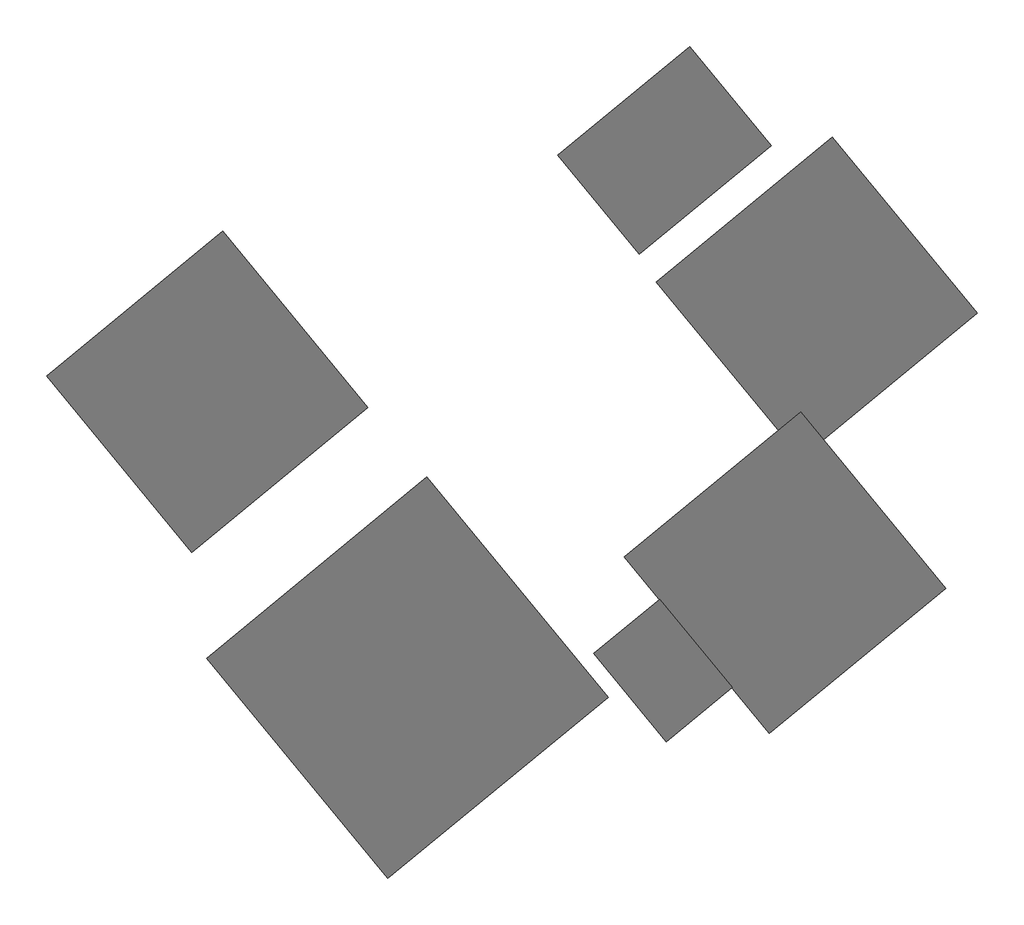
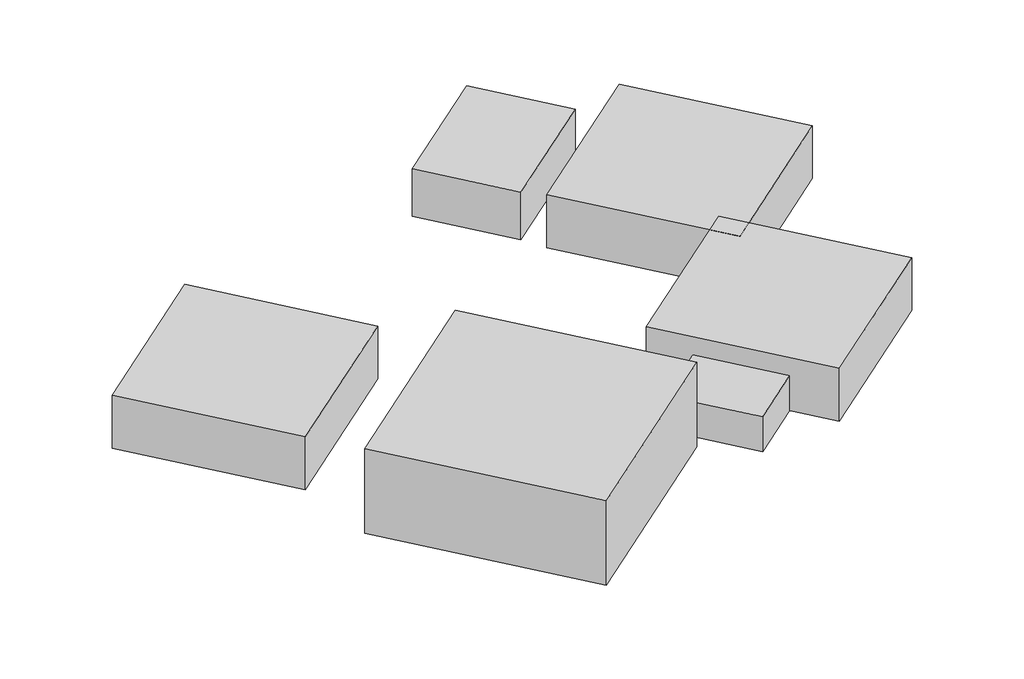
# One storey: 6 proxies.
"""IFC4 building model written with IfcOpenShell, lengths in millimetres."""

from ifc_helpers import new_model, si_unit, frame, origin, place, context, project, spatial, polyline, outline, extrude, element, save

model = new_model("IFC4")

# Units and contexts
model_context = context("Model", 3, world=origin())
ifc_project = project(units=[si_unit("LENGTHUNIT", "METRE", prefix="MILLI")], contexts=[model_context])

# Site, building, storey
site = spatial("IfcSite", under=ifc_project)
building = spatial("IfcBuilding", under=site)
storey = spatial("IfcBuildingStorey", under=building, Name="f3-展厅", Elevation=17500.0)

# Proxies
placement = place(None, origin())
element("IfcBuildingElementProxy", 1, Name="公共-封闭 : Gallery-Big", ObjectType="公共-封闭 : Gallery-Big", at=placement, inside=storey, context=model_context, shape_type="SweptSolid", body=[
    extrude(outline(polyline([(-29475.375386, -24866.8019738), (-42184.0405117, -9423.6860084), (-26740.9245463, 3284.9791173), (-14032.2594206, -12158.1368482), (-29475.375386, -24866.8019738)])), frame((0.0, 0.0, 17500.0), z_axis=(0.0, 0.0, 1.0), x_axis=(1.0, 0.0, 0.0)), (0.0, 0.0, 1.0), 8000.0),
])
element("IfcBuildingElementProxy", 2, Name="公共-封闭 : Gallery-Middle", ObjectType="公共-封闭 : Gallery-Middle", at=placement, inside=storey, context=model_context, shape_type="SweptSolid", body=[
    extrude(outline(polyline([(-492.5871713, 4613.457612), (-10659.5192719, 16967.9503844), (1694.9735005, 27134.8824849), (11861.9056011, 14780.3897125), (-492.5871713, 4613.457612)])), frame((0.0, 0.0, 17500.0), z_axis=(0.0, 0.0, 1.0), x_axis=(1.0, 0.0, 0.0)), (0.0, 0.0, 1.0), 5000.0),
])
element("IfcBuildingElementProxy", 3, Name="公共-封闭 : Gallery-Middle", ObjectType="公共-封闭 : Gallery-Middle", at=placement, inside=storey, context=model_context, shape_type="SweptSolid", body=[
    extrude(outline(polyline([(-2728.7186006, -14686.3227176), (-12895.6507012, -2331.8299452), (-541.1579288, 7835.1021553), (9625.7741718, -4519.3906171), (-2728.7186006, -14686.3227176)])), frame((0.0, 0.0, 17500.0), z_axis=(0.0, 0.0, 1.0), x_axis=(1.0, 0.0, 0.0)), (0.0, 0.0, 1.0), 5000.0),
])
element("IfcBuildingElementProxy", 4, Name="公共-封闭 : Gallery-Middle", ObjectType="公共-封闭 : Gallery-Middle", at=placement, inside=storey, context=model_context, shape_type="SweptSolid", body=[
    extrude(outline(polyline([(-43231.5828584, -1987.7462838), (-53398.514959, 10366.7464885), (-41044.0221866, 20533.6785891), (-30877.0900861, 8179.1858167), (-43231.5828584, -1987.7462838)])), frame((0.0, 0.0, 17500.0), z_axis=(0.0, 0.0, 1.0), x_axis=(1.0, 0.0, 0.0)), (0.0, 0.0, 1.0), 5000.0),
])
element("IfcBuildingElementProxy", 5, Name="公共-封闭 : Gallery-Small", ObjectType="公共-封闭 : Gallery-Small", at=placement, inside=storey, context=model_context, shape_type="SweptSolid", body=[
    extrude(outline(polyline([(-11856.9381005, 18909.0766924), (-17575.8374071, 25858.4788769), (-8309.9678278, 33483.6779523), (-2591.0685212, 26534.2757679), (-11856.9381005, 18909.0766924)])), frame((0.0, 0.0, 17500.0), z_axis=(0.0, 0.0, 1.0), x_axis=(1.0, 0.0, 0.0)), (0.0, 0.0, 1.0), 4500.0),
])
element("IfcBuildingElementProxy", 6, Name="临时私有-封闭 : Restrooms-Gallery-3f", ObjectType="临时私有-封闭 : Restrooms-Gallery-3f", at=placement, inside=storey, context=model_context, shape_type="SweptSolid", body=[
    extrude(outline(polyline([(-5312.0353372, -11458.3253572), (-9944.9701269, -15270.9248949), (-15028.4361772, -9093.6785087), (-10395.5013875, -5281.078971), (-5312.0353372, -11458.3253572)])), frame((0.0, 0.0, 17500.0), z_axis=(0.0, 0.0, 1.0), x_axis=(1.0, 0.0, 0.0)), (0.0, 0.0, 1.0), 3300.0),
])

save(model, "model.ifc")

# Revit data of these elements
# Type "公共-封闭 : Gallery-Big"
#   Default Elevation = 1219.2 mm
#   公共_封闭_房间_面积 = 400.00 m²
#   公共_封闭_房间_进深 = 20000 mm
#   公共_封闭_房间_开间 = 20000 mm
#   公共_封闭_房间_层高 = 8000 mm
# Type "公共-封闭 : Gallery-Middle"
#   Default Elevation = 1219.2 mm
#   公共_封闭_房间_面积 = 256.00 m²
#   公共_封闭_房间_进深 = 16000 mm
#   公共_封闭_房间_开间 = 16000 mm
#   公共_封闭_房间_层高 = 5000 mm
# Type "公共-封闭 : Gallery-Small"
#   Default Elevation = 1219.2 mm
#   公共_封闭_房间_面积 = 108.00 m²
#   公共_封闭_房间_进深 = 9000 mm
#   公共_封闭_房间_开间 = 12000 mm
#   公共_封闭_房间_层高 = 4500 mm
# Type "临时私有-封闭 : Restrooms-Gallery-3f"
#   Default Elevation = 1219.2 mm
#   临时私有_封闭_房间_面积 = 48.00 m²
#   临时私有_封闭_房间_进深 = 6000 mm
#   临时私有_封闭_房间_开间 = 8000 mm
#   临时私有_封闭_房间_层高 = 3300 mm
# Element 1 (IfcBuildingElementProxy, "公共-封闭 : Gallery-Big")
#   Phase Created = 新构造
#   Materials on its faces: "公共_封闭_房间"
# Elements 2, 3, 4 (IfcBuildingElementProxy, "公共-封闭 : Gallery-Middle")
#   Phase Created = 新构造
#   Materials on its faces: "公共_封闭_房间"
# Element 5 (IfcBuildingElementProxy, "公共-封闭 : Gallery-Small")
#   Phase Created = 新构造
#   Materials on its faces: "公共_封闭_房间"
# Element 6 (IfcBuildingElementProxy, "临时私有-封闭 : Restrooms-Gallery-3f")
#   Phase Created = 新构造
#   Materials on its faces: "临时私有_封闭_房间"
# Materials
#   "公共_封闭_房间": class "其他", colour RGB 135 60 10, transparency 0
#   "临时私有_封闭_房间": class "其他", colour RGB 77 38 0, transparency 0
